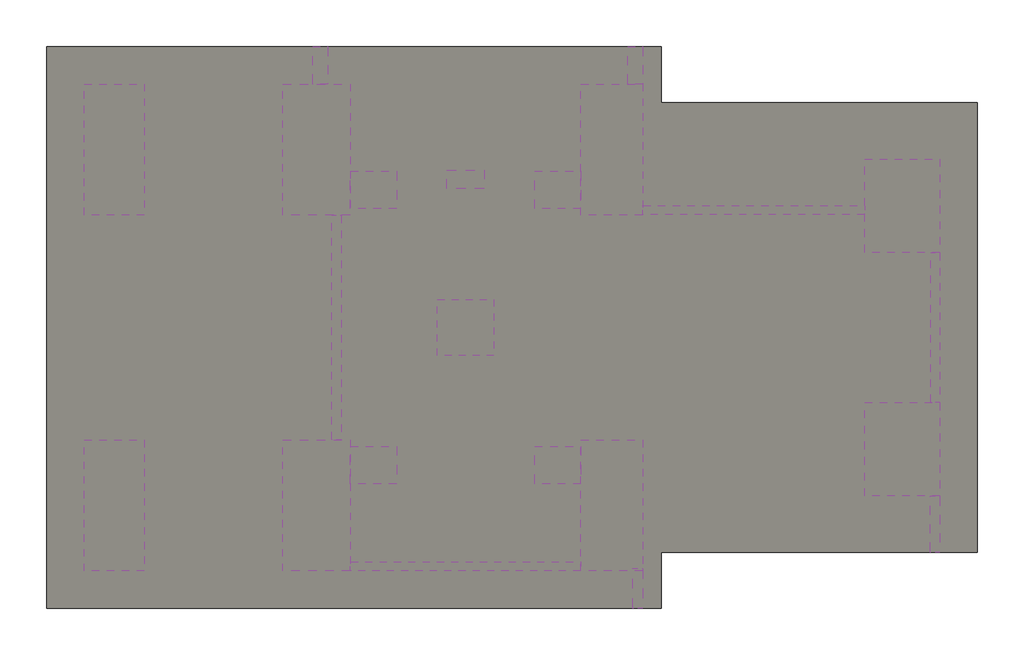
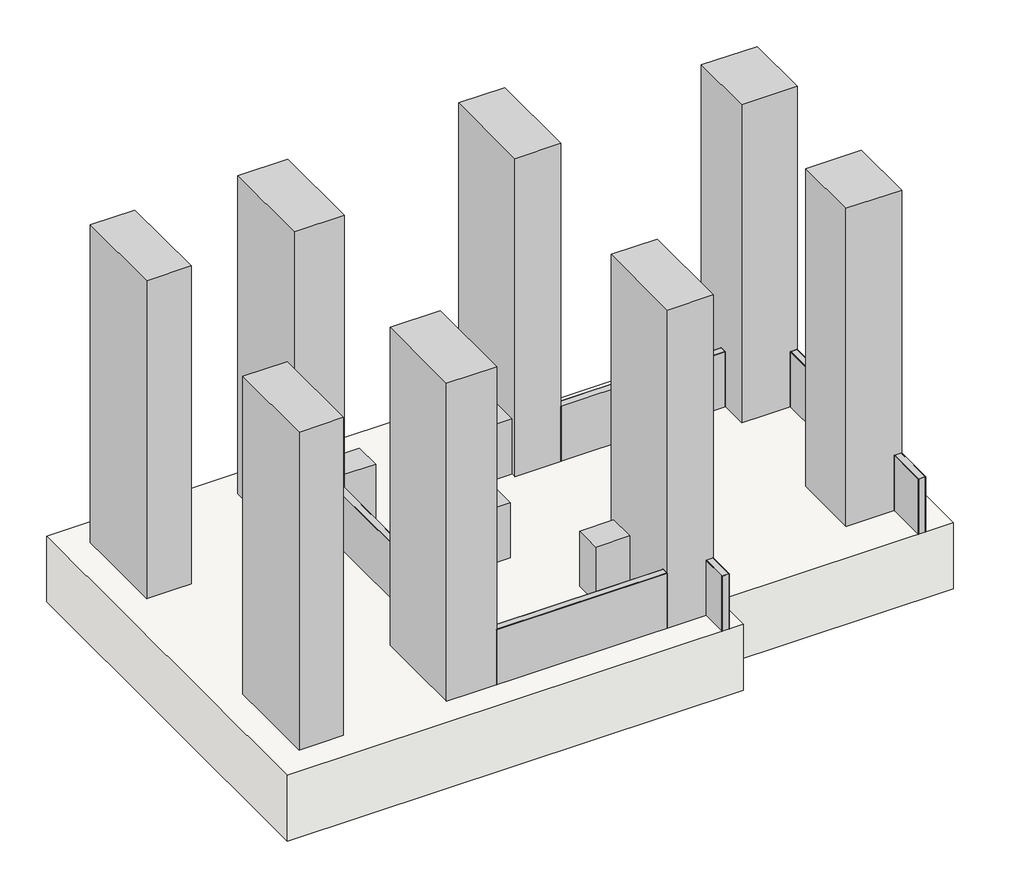
# One storey: 14 columns, 8 beams, 1 slab.
# Revit data of these elements (continued)
# Room at (7378.019, 15859.507) mm, phase "New Construction", upper level "G.L", upper offset 2700 mm, lower offset 0 mm (continued)
#   Wall Finish = "LATEX PAINT ON THK.15 CEMENT PLASTER + MASONRY WALL"
#   Floor Finish = "PVC TILE W/ADHESIVE ON STEEL TROWELED CONC. SLAB"
#   Number = "UYF01R0002"
#   Name = "RECEPTION WAITING ROOM"
#   F01) Building Name = "MAIN GATE SECURITY BUILDING"
#   S01) Room Name = "RECEPTION WAITING ROOM"
#   S02) Room Number(Project) = "UYF01R0002"
#   S03) Floor = "GF"
#   S04) Level = "FL+0"
#   S11) Space by Function_Lv1 = "Space for Architecture"
#   S12) Space by Function_Lv2 = "Commerce Activity Spaces"
#   S13) Space by Function_Lv3 = "Reception Space"
#   S21) Space by Form = "Enclosed"
# Room, not placed, phase "New Construction", upper offset 0 mm, lower offset 0 mm
#   Comments = ""
#   Base Finish = "EXPOXY PAINT ON THK.15 CEMENT PLASTER(H=100)"
#   Ceiling Finish = "LATEX PAINT ON FAIR FACED CONC."
#   Wall Finish = "LATEX PAINT ON THK.15 CEMENT PLASTER + MASONRY WALL"
#   Floor Finish = "EPOXY PAINT ON STEEL TROWELED CONC. SLAB"
#   Number = "1"
#   Name = ""
#   F01) Building Name = "CENTRAL CONTROL BUILDING"
#   S01) Room Name = "CABLE ROOM"
#   S02) Room Number(Project) = "UCA01R0001"
# Room, not placed, phase "New Construction", upper offset 0 mm, lower offset 0 mm
#   Comments = ""
#   Number = "2"
#   Name = ""
#   S01) Room Name = ""
#   S02) Room Number(Project) = ""
